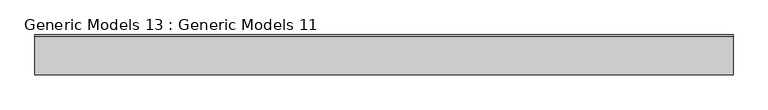
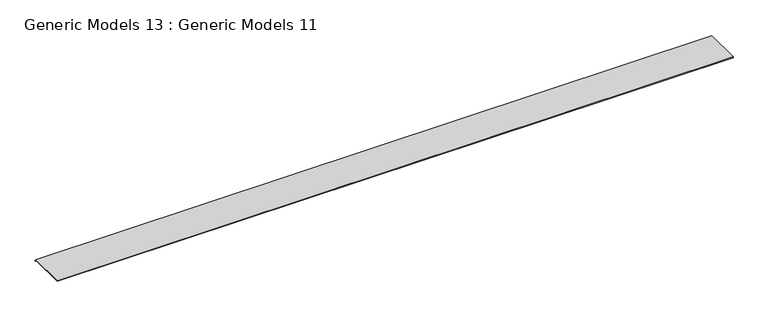
"""IFC4 building model written with IfcOpenShell, lengths in millimetres: proxy geometry, Generic Models 13 : Generic Models 11."""

from ifc_helpers import new_model, si_unit, frame, origin, place, context, project, spatial, polyline, outline, extrude, source, transform, mapped, element, save


def generic_models_13_generic_models_11_74c8020a(model_context):
    return source(origin(), model_context, "Body", "SweptSolid", [
        extrude(outline(polyline([(40907.0387657, 268878.05), (40907.0387657, 268879.6375), (40995.1450157, 268879.6375), (40999.6351438, 268875.1473719), (40998.5126118, 268874.0248399), (40994.4874517, 268878.05), (40907.0387657, 268878.05)])), frame((26424.3233872, 0.0, 0.0), z_axis=(1.0, 0.0, 0.0), x_axis=(0.0, 1.0, 0.0)), (0.0, 0.0, 1.0), 1629.052575),
    ])


if __name__ == "__main__":
    model = new_model("IFC4")
    model_context = context("Model", 3, world=origin())
    ifc_project = project(units=[si_unit("LENGTHUNIT", "METRE", prefix="MILLI")], contexts=[model_context])
    site = spatial("IfcSite", under=ifc_project)
    building = spatial("IfcBuilding", under=site)
    placement = place(None, origin())
    generic_models_13_generic_models_11_shape = generic_models_13_generic_models_11_74c8020a(model_context)
    element("IfcBuildingElementProxy", 1, Name="Generic Models 13 : Generic Models 11", ObjectType="Generic Models 13 : Generic Models 11", at=placement, inside=building, context=model_context, shape_type="MappedRepresentation", body=[
        mapped(generic_models_13_generic_models_11_shape, transform((0.0, 0.0, 0.0), x_axis=(1.0, 0.0, 0.0), y_axis=(0.0, 1.0, 0.0), z_axis=(0.0, 0.0, 1.0))),
    ])
    save(model, "model.ifc")

# Revit data of these elements
# Element 1 (IfcBuildingElementProxy, "Generic Models 13 : Generic Models 11")
#   Materials on its faces: "GALV. BRAKE METAL - (COLOR: GALV.)"
# Materials
#   "GALV. BRAKE METAL - (COLOR: GALV.)": class "Generic", colour RGB 234 234 234, transparency 0, Cost = 0
